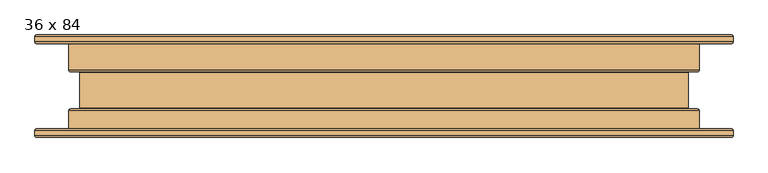
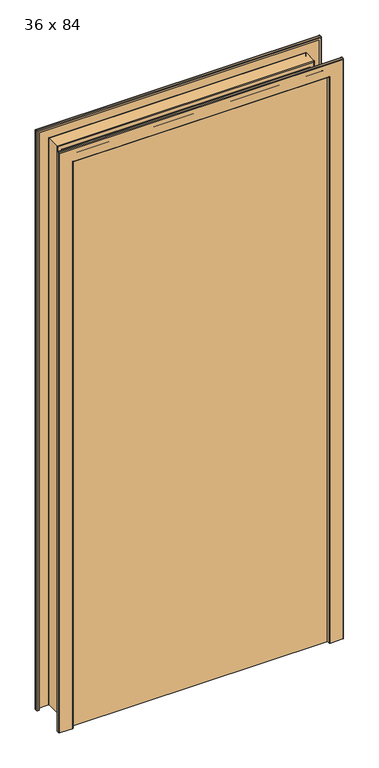
"""IFC4 building model written with IfcOpenShell, lengths in millimetres: door geometry, Door-Dunbarton_Doors-Hollow_Metal_Core : 36 x 84."""

from ifc_helpers import new_model, si_unit, frame, origin, origin_with_axes, place, context, project, spatial, polyline, circle_curve, ellipse_curve, outline, extrude, source, transform, mapped, element, save
from ifc_brep_helpers import plane_surface, cylinder_surface, revolved_surface, advanced_brep


def door_36_x_84_91fbd793(model_context):
    return source(origin(), model_context, "Body", "SolidModel", [
        advanced_brep(
        [(-505.42825, 61.976, 0.0), (-508.0, 64.54775, 0.0), (-508.0, 72.0725, 0.0), (-505.42825, 74.64425, 0.0), (-459.77175, 74.64425, 0.0), (-457.2, 72.0725, 0.0), (-457.2, 23.27275, 0.0), (-456.184, 22.25675, 0.0), (-443.89675, 22.25675, 0.0), (-441.325, 19.685, 0.0), (-441.325, -32.1056, 0.0), (-443.89675, -34.67735, 0.0), (-456.184, -34.67735, 0.0), (-457.2, -35.69335, 0.0), (-457.2, -72.009, 0.0), (-459.77175, -74.58075, 0.0), (-505.42825, -74.58075, 0.0), (-508.0, -72.009, 0.0), (-508.0, -64.48425, 0.0), (-505.42825, -61.9125, 0.0), (-500.0625, -61.9125, 0.0), (-500.0625, -63.46825, 0.0), (-505.42825, -63.46825, 0.0), (-506.44425, -64.48425, 0.0), (-506.44425, -72.009, 0.0), (-505.42825, -73.025, 0.0), (-459.77175, -73.025, 0.0), (-458.75575, -72.009, 0.0), (-458.75575, -35.69335, 0.0), (-456.184, -33.1216, 0.0), (-443.89675, -33.1216, 0.0), (-442.88075, -32.1056, 0.0), (-442.88075, 19.685, 0.0), (-443.89675, 20.701, 0.0), (-456.184, 20.701, 0.0), (-458.75575, 23.27275, 0.0), (-458.75575, 72.0725, 0.0), (-459.77175, 73.0885, 0.0), (-505.42825, 73.0885, 0.0), (-506.44425, 72.0725, 0.0), (-506.44425, 64.54775, 0.0), (-505.42825, 63.53175, 0.0), (-500.0625, 63.53175, 0.0), (-500.0625, 61.976, 0.0), (-505.42825, 61.976, 2181.82825), (-508.0, 64.54775, 2184.4), (-508.0, 72.0725, 2184.4), (-505.42825, 74.64425, 2181.82825), (505.42825, 74.64425, 2181.82825), (505.42825, 74.64425, 0.0), (459.77175, 74.64425, 0.0), (459.77175, 74.64425, 2136.17175), (-459.77175, 74.64425, 2136.17175), (-457.2, 72.0725, 2133.6), (-457.2, 23.27275, 2133.6), (-456.184, 22.25675, 2132.584), (456.184, 22.25675, 2132.584), (456.184, 22.25675, 0.0), (443.89675, 22.25675, 0.0), (443.89675, 22.25675, 2120.29675), (-443.89675, 22.25675, 2120.29675), (-441.325, 19.685, 2117.725), (-441.325, -32.1056, 2117.725), (-443.89675, -34.67735, 2120.29675), (443.89675, -34.67735, 2120.29675), (443.89675, -34.67735, 0.0), (456.184, -34.67735, 0.0), (456.184, -34.67735, 2132.584), (-456.184, -34.67735, 2132.584), (-457.2, -35.69335, 2133.6), (-457.2, -72.009, 2133.6), (-459.77175, -74.58075, 2136.17175), (459.77175, -74.58075, 2136.17175), (459.77175, -74.58075, 0.0), (505.42825, -74.58075, 0.0), (505.42825, -74.58075, 2181.82825), (-505.42825, -74.58075, 2181.82825), (-508.0, -72.009, 2184.4), (-508.0, -64.48425, 2184.4), (-505.42825, -61.9125, 2181.82825), (505.42825, -61.9125, 2181.82825), (505.42825, -61.9125, 0.0), (500.0625, -61.9125, 0.0), (500.0625, -61.9125, 2176.4625), (-500.0625, -61.9125, 2176.4625), (-500.0625, -63.46825, 2176.4625), (500.0625, -63.46825, 2176.4625), (500.0625, -63.46825, 0.0), (505.42825, -63.46825, 0.0), (505.42825, -63.46825, 2181.82825), (-505.42825, -63.46825, 2181.82825), (-506.44425, -64.48425, 2182.84425), (-506.44425, -72.009, 2182.84425), (-505.42825, -73.025, 2181.82825), (505.42825, -73.025, 2181.82825), (505.42825, -73.025, 0.0), (459.77175, -73.025, 0.0), (459.77175, -73.025, 2136.17175), (-459.77175, -73.025, 2136.17175), (-458.75575, -72.009, 2135.15575), (-458.75575, -35.69335, 2135.15575), (-456.184, -33.1216, 2132.584), (456.184, -33.1216, 2132.584), (456.184, -33.1216, 0.0), (443.89675, -33.1216, 0.0), (443.89675, -33.1216, 2120.29675), (-443.89675, -33.1216, 2120.29675), (-442.88075, -32.1056, 2119.28075), (-442.88075, 19.685, 2119.28075), (-443.89675, 20.701, 2120.29675), (443.89675, 20.701, 2120.29675), (443.89675, 20.701, 0.0), (456.184, 20.701, 0.0), (456.184, 20.701, 2132.584), (-456.184, 20.701, 2132.584), (-458.75575, 23.27275, 2135.15575), (-458.75575, 72.0725, 2135.15575), (-459.77175, 73.0885, 2136.17175), (459.77175, 73.0885, 2136.17175), (459.77175, 73.0885, 0.0), (505.42825, 73.0885, 0.0), (505.42825, 73.0885, 2181.82825), (-505.42825, 73.0885, 2181.82825), (-506.44425, 72.0725, 2182.84425), (-506.44425, 64.54775, 2182.84425), (-505.42825, 63.53175, 2181.82825), (505.42825, 63.53175, 2181.82825), (505.42825, 63.53175, 0.0), (500.0625, 63.53175, 0.0), (500.0625, 63.53175, 2176.4625), (-500.0625, 63.53175, 2176.4625), (-500.0625, 61.976, 2176.4625), (500.0625, 61.976, 2176.4625), (500.0625, 61.976, 0.0), (505.42825, 61.976, 0.0), (505.42825, 61.976, 2181.82825), (508.0, 64.54775, 2184.4), (508.0, 72.0725, 2184.4), (457.2, 72.0725, 2133.6), (457.2, 23.27275, 2133.6), (441.325, 19.685, 2117.725), (441.325, -32.1056, 2117.725), (457.2, -35.69335, 2133.6), (457.2, -72.009, 2133.6), (508.0, -72.009, 2184.4), (508.0, -64.48425, 2184.4), (506.44425, -64.48425, 2182.84425), (506.44425, -72.009, 2182.84425), (458.75575, -72.009, 2135.15575), (458.75575, -35.69335, 2135.15575), (442.88075, -32.1056, 2119.28075), (442.88075, 19.685, 2119.28075), (458.75575, 23.27275, 2135.15575), (458.75575, 72.0725, 2135.15575), (506.44425, 72.0725, 2182.84425), (506.44425, 64.54775, 2182.84425), (506.44425, 64.54775, 0.0), (506.44425, 72.0725, 0.0), (458.75575, 72.0725, 0.0), (458.75575, 23.27275, 0.0), (442.88075, 19.685, 0.0), (442.88075, -32.1056, 0.0), (458.75575, -35.69335, 0.0), (458.75575, -72.009, 0.0), (506.44425, -72.009, 0.0), (506.44425, -64.48425, 0.0), (508.0, -64.48425, 0.0), (508.0, -72.009, 0.0), (457.2, -72.009, 0.0), (457.2, -35.69335, 0.0), (441.325, -32.1056, 0.0), (441.325, 19.685, 0.0), (457.2, 23.27275, 0.0), (457.2, 72.0725, 0.0), (508.0, 72.0725, 0.0), (508.0, 64.54775, 0.0)],
        [
            (0, 1, circle_curve(frame((-505.42825, 64.54775, 0.0), z_axis=(0.0, 0.0, -1.0), x_axis=(0.0, -1.0, 0.0)), 2.57175)),
            (1, 2),
            (2, 3, circle_curve(frame((-505.42825, 72.0725, 0.0), z_axis=(0.0, 0.0, -1.0), x_axis=(0.0, -1.0, 0.0)), 2.57175)),
            (3, 4),
            (4, 5, circle_curve(frame((-459.77175, 72.0725, 0.0), z_axis=(0.0, 0.0, -1.0), x_axis=(0.0, -1.0, 0.0)), 2.57175)),
            (5, 6),
            (6, 7, circle_curve(frame((-456.184, 23.27275, 0.0), z_axis=(0.0, 0.0, 1.0), x_axis=(0.0, -1.0, 0.0)), 1.016)),
            (7, 8),
            (8, 9, circle_curve(frame((-443.89675, 19.685, 0.0), z_axis=(0.0, 0.0, -1.0), x_axis=(0.0, -1.0, 0.0)), 2.57175)),
            (9, 10),
            (10, 11, circle_curve(frame((-443.89675, -32.1056, 0.0), z_axis=(0.0, 0.0, -1.0), x_axis=(0.0, -1.0, 0.0)), 2.57175)),
            (11, 12),
            (12, 13, circle_curve(frame((-456.184, -35.69335, 0.0), z_axis=(0.0, 0.0, 1.0), x_axis=(0.0, -1.0, 0.0)), 1.016)),
            (13, 14),
            (14, 15, circle_curve(frame((-459.77175, -72.009, 0.0), z_axis=(0.0, 0.0, -1.0), x_axis=(0.0, -1.0, 0.0)), 2.57175)),
            (15, 16),
            (16, 17, circle_curve(frame((-505.42825, -72.009, 0.0), z_axis=(0.0, 0.0, -1.0), x_axis=(0.0, -1.0, 0.0)), 2.57175)),
            (17, 18),
            (18, 19, circle_curve(frame((-505.42825, -64.48425, 0.0), z_axis=(0.0, 0.0, -1.0), x_axis=(0.0, -1.0, 0.0)), 2.57175)),
            (19, 20),
            (20, 21),
            (21, 22),
            (22, 23, circle_curve(frame((-505.42825, -64.48425, 0.0), z_axis=(0.0, 0.0, 1.0), x_axis=(0.0, -1.0, 0.0)), 1.016)),
            (23, 24),
            (24, 25, circle_curve(frame((-505.42825, -72.009, 0.0), z_axis=(0.0, 0.0, 1.0), x_axis=(0.0, -1.0, 0.0)), 1.016)),
            (25, 26),
            (26, 27, circle_curve(frame((-459.77175, -72.009, 0.0), z_axis=(0.0, 0.0, 1.0), x_axis=(0.0, -1.0, 0.0)), 1.016)),
            (27, 28),
            (28, 29, circle_curve(frame((-456.184, -35.69335, 0.0), z_axis=(0.0, 0.0, -1.0), x_axis=(0.0, -1.0, 0.0)), 2.57175)),
            (29, 30),
            (30, 31, circle_curve(frame((-443.89675, -32.1056, 0.0), z_axis=(0.0, 0.0, 1.0), x_axis=(0.0, -1.0, 0.0)), 1.016)),
            (31, 32),
            (32, 33, circle_curve(frame((-443.89675, 19.685, 0.0), z_axis=(0.0, 0.0, 1.0), x_axis=(0.0, -1.0, 0.0)), 1.016)),
            (33, 34),
            (34, 35, circle_curve(frame((-456.184, 23.27275, 0.0), z_axis=(0.0, 0.0, -1.0), x_axis=(0.0, -1.0, 0.0)), 2.57175)),
            (35, 36),
            (36, 37, circle_curve(frame((-459.77175, 72.0725, 0.0), z_axis=(0.0, 0.0, 1.0), x_axis=(0.0, -1.0, 0.0)), 1.016)),
            (37, 38),
            (38, 39, circle_curve(frame((-505.42825, 72.0725, 0.0), z_axis=(0.0, 0.0, 1.0), x_axis=(0.0, -1.0, 0.0)), 1.016)),
            (39, 40),
            (40, 41, circle_curve(frame((-505.42825, 64.54775, 0.0), z_axis=(0.0, 0.0, 1.0), x_axis=(0.0, -1.0, 0.0)), 1.016)),
            (41, 42),
            (42, 43),
            (43, 0),
            (0, 44),
            (44, 45, ellipse_curve(frame((-505.42825, 64.54775, 2181.82825), z_axis=(-0.7071067811865475, 0.0, -0.7071067811865475), x_axis=(0.7071067811865474, 0.0, -0.7071067811865476)), 3.6370037, 2.57175)),
            (45, 1),
            (45, 46),
            (46, 2),
            (46, 47, ellipse_curve(frame((-505.42825, 72.0725, 2181.82825), z_axis=(-0.7071067811865475, 0.0, -0.7071067811865475), x_axis=(0.7071067811865474, 0.0, -0.7071067811865476)), 3.6370037, 2.57175)),
            (47, 3),
            (47, 48),
            (48, 49),
            (49, 50),
            (50, 51),
            (51, 52),
            (52, 4),
            (52, 53, ellipse_curve(frame((-459.77175, 72.0725, 2136.17175), z_axis=(-0.7071067811865475, 0.0, -0.7071067811865475), x_axis=(0.7071067811865474, 0.0, -0.7071067811865476)), 3.6370037, 2.57175)),
            (53, 5),
            (53, 54),
            (54, 6),
            (54, 55, ellipse_curve(frame((-456.184, 23.27275, 2132.584), z_axis=(0.7071067811865475, 0.0, 0.7071067811865475), x_axis=(-0.7071067811865474, 0.0, 0.7071067811865476)), 1.436841, 1.016)),
            (55, 7),
            (55, 56),
            (56, 57),
            (57, 58),
            (58, 59),
            (59, 60),
            (60, 8),
            (60, 61, ellipse_curve(frame((-443.89675, 19.685, 2120.29675), z_axis=(-0.7071067811865475, 0.0, -0.7071067811865475), x_axis=(0.7071067811865474, 0.0, -0.7071067811865476)), 3.6370037, 2.57175)),
            (61, 9),
            (61, 62),
            (62, 10),
            (62, 63, ellipse_curve(frame((-443.89675, -32.1056, 2120.29675), z_axis=(-0.7071067811865475, 0.0, -0.7071067811865475), x_axis=(0.7071067811865474, 0.0, -0.7071067811865476)), 3.6370037, 2.57175)),
            (63, 11),
            (63, 64),
            (64, 65),
            (65, 66),
            (66, 67),
            (67, 68),
            (68, 12),
            (68, 69, ellipse_curve(frame((-456.184, -35.69335, 2132.584), z_axis=(0.7071067811865475, 0.0, 0.7071067811865475), x_axis=(-0.7071067811865474, 0.0, 0.7071067811865476)), 1.436841, 1.016)),
            (69, 13),
            (69, 70),
            (70, 14),
            (70, 71, ellipse_curve(frame((-459.77175, -72.009, 2136.17175), z_axis=(-0.7071067811865475, 0.0, -0.7071067811865475), x_axis=(0.7071067811865474, 0.0, -0.7071067811865476)), 3.6370037, 2.57175)),
            (71, 15),
            (71, 72),
            (72, 73),
            (73, 74),
            (74, 75),
            (75, 76),
            (76, 16),
            (76, 77, ellipse_curve(frame((-505.42825, -72.009, 2181.82825), z_axis=(-0.7071067811865475, 0.0, -0.7071067811865475), x_axis=(0.7071067811865474, 0.0, -0.7071067811865476)), 3.6370037, 2.57175)),
            (77, 17),
            (77, 78),
            (78, 18),
            (78, 79, ellipse_curve(frame((-505.42825, -64.48425, 2181.82825), z_axis=(-0.7071067811865475, 0.0, -0.7071067811865475), x_axis=(0.7071067811865474, 0.0, -0.7071067811865476)), 3.6370037, 2.57175)),
            (79, 19),
            (79, 80),
            (80, 81),
            (81, 82),
            (82, 83),
            (83, 84),
            (84, 20),
            (84, 85),
            (85, 21),
            (85, 86),
            (86, 87),
            (87, 88),
            (88, 89),
            (89, 90),
            (90, 22),
            (90, 91, ellipse_curve(frame((-505.42825, -64.48425, 2181.82825), z_axis=(0.7071067811865475, 0.0, 0.7071067811865475), x_axis=(-0.7071067811865474, 0.0, 0.7071067811865476)), 1.436841, 1.016)),
            (91, 23),
            (91, 92),
            (92, 24),
            (92, 93, ellipse_curve(frame((-505.42825, -72.009, 2181.82825), z_axis=(0.7071067811865475, 0.0, 0.7071067811865475), x_axis=(-0.7071067811865474, 0.0, 0.7071067811865476)), 1.436841, 1.016)),
            (93, 25),
            (93, 94),
            (94, 95),
            (95, 96),
            (96, 97),
            (97, 98),
            (98, 26),
            (98, 99, ellipse_curve(frame((-459.77175, -72.009, 2136.17175), z_axis=(0.7071067811865475, 0.0, 0.7071067811865475), x_axis=(-0.7071067811865474, 0.0, 0.7071067811865476)), 1.436841, 1.016)),
            (99, 27),
            (99, 100),
            (100, 28),
            (100, 101, ellipse_curve(frame((-456.184, -35.69335, 2132.584), z_axis=(-0.7071067811865475, 0.0, -0.7071067811865475), x_axis=(0.7071067811865474, 0.0, -0.7071067811865476)), 3.6370037, 2.57175)),
            (101, 29),
            (101, 102),
            (102, 103),
            (103, 104),
            (104, 105),
            (105, 106),
            (106, 30),
            (106, 107, ellipse_curve(frame((-443.89675, -32.1056, 2120.29675), z_axis=(0.7071067811865475, 0.0, 0.7071067811865475), x_axis=(-0.7071067811865474, 0.0, 0.7071067811865476)), 1.436841, 1.016)),
            (107, 31),
            (107, 108),
            (108, 32),
            (108, 109, ellipse_curve(frame((-443.89675, 19.685, 2120.29675), z_axis=(0.7071067811865475, 0.0, 0.7071067811865475), x_axis=(-0.7071067811865474, 0.0, 0.7071067811865476)), 1.436841, 1.016)),
            (109, 33),
            (109, 110),
            (110, 111),
            (111, 112),
            (112, 113),
            (113, 114),
            (114, 34),
            (114, 115, ellipse_curve(frame((-456.184, 23.27275, 2132.584), z_axis=(-0.7071067811865475, 0.0, -0.7071067811865475), x_axis=(0.7071067811865474, 0.0, -0.7071067811865476)), 3.6370037, 2.57175)),
            (115, 35),
            (115, 116),
            (116, 36),
            (116, 117, ellipse_curve(frame((-459.77175, 72.0725, 2136.17175), z_axis=(0.7071067811865475, 0.0, 0.7071067811865475), x_axis=(-0.7071067811865474, 0.0, 0.7071067811865476)), 1.436841, 1.016)),
            (117, 37),
            (117, 118),
            (118, 119),
            (119, 120),
            (120, 121),
            (121, 122),
            (122, 38),
            (122, 123, ellipse_curve(frame((-505.42825, 72.0725, 2181.82825), z_axis=(0.7071067811865475, 0.0, 0.7071067811865475), x_axis=(-0.7071067811865474, 0.0, 0.7071067811865476)), 1.436841, 1.016)),
            (123, 39),
            (123, 124),
            (124, 40),
            (124, 125, ellipse_curve(frame((-505.42825, 64.54775, 2181.82825), z_axis=(0.7071067811865475, 0.0, 0.7071067811865475), x_axis=(-0.7071067811865474, 0.0, 0.7071067811865476)), 1.436841, 1.016)),
            (125, 41),
            (125, 126),
            (126, 127),
            (127, 128),
            (128, 129),
            (129, 130),
            (130, 42),
            (130, 131),
            (131, 43),
            (131, 132),
            (132, 133),
            (133, 134),
            (134, 135),
            (135, 44),
            (135, 136, ellipse_curve(frame((505.42825, 64.54775, 2181.82825), z_axis=(-0.7071067811865475, 0.0, 0.7071067811865475), x_axis=(-0.7071067811865476, 0.0, -0.7071067811865474)), 3.6370037, 2.57175)),
            (136, 45),
            (136, 137),
            (137, 46),
            (137, 48, ellipse_curve(frame((505.42825, 72.0725, 2181.82825), z_axis=(-0.7071067811865475, 0.0, 0.7071067811865475), x_axis=(-0.7071067811865476, 0.0, -0.7071067811865474)), 3.6370037, 2.57175)),
            (51, 138, ellipse_curve(frame((459.77175, 72.0725, 2136.17175), z_axis=(-0.7071067811865475, 0.0, 0.7071067811865475), x_axis=(-0.7071067811865476, 0.0, -0.7071067811865474)), 3.6370037, 2.57175)),
            (138, 53),
            (138, 139),
            (139, 54),
            (139, 56, ellipse_curve(frame((456.184, 23.27275, 2132.584), z_axis=(0.7071067811865475, 0.0, -0.7071067811865475), x_axis=(0.7071067811865476, 0.0, 0.7071067811865474)), 1.436841, 1.016)),
            (59, 140, ellipse_curve(frame((443.89675, 19.685, 2120.29675), z_axis=(-0.7071067811865475, 0.0, 0.7071067811865475), x_axis=(-0.7071067811865476, 0.0, -0.7071067811865474)), 3.6370037, 2.57175)),
            (140, 61),
            (140, 141),
            (141, 62),
            (141, 64, ellipse_curve(frame((443.89675, -32.1056, 2120.29675), z_axis=(-0.7071067811865475, 0.0, 0.7071067811865475), x_axis=(-0.7071067811865476, 0.0, -0.7071067811865474)), 3.6370037, 2.57175)),
            (67, 142, ellipse_curve(frame((456.184, -35.69335, 2132.584), z_axis=(0.7071067811865475, 0.0, -0.7071067811865475), x_axis=(0.7071067811865476, 0.0, 0.7071067811865474)), 1.436841, 1.016)),
            (142, 69),
            (142, 143),
            (143, 70),
            (143, 72, ellipse_curve(frame((459.77175, -72.009, 2136.17175), z_axis=(-0.7071067811865475, 0.0, 0.7071067811865475), x_axis=(-0.7071067811865476, 0.0, -0.7071067811865474)), 3.6370037, 2.57175)),
            (75, 144, ellipse_curve(frame((505.42825, -72.009, 2181.82825), z_axis=(-0.7071067811865475, 0.0, 0.7071067811865475), x_axis=(-0.7071067811865476, 0.0, -0.7071067811865474)), 3.6370037, 2.57175)),
            (144, 77),
            (144, 145),
            (145, 78),
            (145, 80, ellipse_curve(frame((505.42825, -64.48425, 2181.82825), z_axis=(-0.7071067811865475, 0.0, 0.7071067811865475), x_axis=(-0.7071067811865476, 0.0, -0.7071067811865474)), 3.6370037, 2.57175)),
            (83, 86),
            (89, 146, ellipse_curve(frame((505.42825, -64.48425, 2181.82825), z_axis=(0.7071067811865475, 0.0, -0.7071067811865475), x_axis=(0.7071067811865476, 0.0, 0.7071067811865474)), 1.436841, 1.016)),
            (146, 91),
            (146, 147),
            (147, 92),
            (147, 94, ellipse_curve(frame((505.42825, -72.009, 2181.82825), z_axis=(0.7071067811865475, 0.0, -0.7071067811865475), x_axis=(0.7071067811865476, 0.0, 0.7071067811865474)), 1.436841, 1.016)),
            (97, 148, ellipse_curve(frame((459.77175, -72.009, 2136.17175), z_axis=(0.7071067811865475, 0.0, -0.7071067811865475), x_axis=(0.7071067811865476, 0.0, 0.7071067811865474)), 1.436841, 1.016)),
            (148, 99),
            (148, 149),
            (149, 100),
            (149, 102, ellipse_curve(frame((456.184, -35.69335, 2132.584), z_axis=(-0.7071067811865475, 0.0, 0.7071067811865475), x_axis=(-0.7071067811865476, 0.0, -0.7071067811865474)), 3.6370037, 2.57175)),
            (105, 150, ellipse_curve(frame((443.89675, -32.1056, 2120.29675), z_axis=(0.7071067811865475, 0.0, -0.7071067811865475), x_axis=(0.7071067811865476, 0.0, 0.7071067811865474)), 1.436841, 1.016)),
            (150, 107),
            (150, 151),
            (151, 108),
            (151, 110, ellipse_curve(frame((443.89675, 19.685, 2120.29675), z_axis=(0.7071067811865475, 0.0, -0.7071067811865475), x_axis=(0.7071067811865476, 0.0, 0.7071067811865474)), 1.436841, 1.016)),
            (113, 152, ellipse_curve(frame((456.184, 23.27275, 2132.584), z_axis=(-0.7071067811865475, 0.0, 0.7071067811865475), x_axis=(-0.7071067811865476, 0.0, -0.7071067811865474)), 3.6370037, 2.57175)),
            (152, 115),
            (152, 153),
            (153, 116),
            (153, 118, ellipse_curve(frame((459.77175, 72.0725, 2136.17175), z_axis=(0.7071067811865475, 0.0, -0.7071067811865475), x_axis=(0.7071067811865476, 0.0, 0.7071067811865474)), 1.436841, 1.016)),
            (121, 154, ellipse_curve(frame((505.42825, 72.0725, 2181.82825), z_axis=(0.7071067811865475, 0.0, -0.7071067811865475), x_axis=(0.7071067811865476, 0.0, 0.7071067811865474)), 1.436841, 1.016)),
            (154, 123),
            (154, 155),
            (155, 124),
            (155, 126, ellipse_curve(frame((505.42825, 64.54775, 2181.82825), z_axis=(0.7071067811865475, 0.0, -0.7071067811865475), x_axis=(0.7071067811865476, 0.0, 0.7071067811865474)), 1.436841, 1.016)),
            (129, 132),
            (133, 128),
            (127, 156, circle_curve(frame((505.42825, 64.54775, 0.0), z_axis=(0.0, 0.0, 1.0), x_axis=(0.0, -1.0, 0.0)), 1.016)),
            (156, 157),
            (157, 120, circle_curve(frame((505.42825, 72.0725, 0.0), z_axis=(0.0, 0.0, 1.0), x_axis=(0.0, -1.0, 0.0)), 1.016)),
            (119, 158, circle_curve(frame((459.77175, 72.0725, 0.0), z_axis=(0.0, 0.0, 1.0), x_axis=(0.0, -1.0, 0.0)), 1.016)),
            (158, 159),
            (159, 112, circle_curve(frame((456.184, 23.27275, 0.0), z_axis=(0.0, 0.0, -1.0), x_axis=(0.0, -1.0, 0.0)), 2.57175)),
            (111, 160, circle_curve(frame((443.89675, 19.685, 0.0), z_axis=(0.0, 0.0, 1.0), x_axis=(0.0, -1.0, 0.0)), 1.016)),
            (160, 161),
            (161, 104, circle_curve(frame((443.89675, -32.1056, 0.0), z_axis=(0.0, 0.0, 1.0), x_axis=(0.0, -1.0, 0.0)), 1.016)),
            (103, 162, circle_curve(frame((456.184, -35.69335, 0.0), z_axis=(0.0, 0.0, -1.0), x_axis=(0.0, -1.0, 0.0)), 2.57175)),
            (162, 163),
            (163, 96, circle_curve(frame((459.77175, -72.009, 0.0), z_axis=(0.0, 0.0, 1.0), x_axis=(0.0, -1.0, 0.0)), 1.016)),
            (95, 164, circle_curve(frame((505.42825, -72.009, 0.0), z_axis=(0.0, 0.0, 1.0), x_axis=(0.0, -1.0, 0.0)), 1.016)),
            (164, 165),
            (165, 88, circle_curve(frame((505.42825, -64.48425, 0.0), z_axis=(0.0, 0.0, 1.0), x_axis=(0.0, -1.0, 0.0)), 1.016)),
            (87, 82),
            (81, 166, circle_curve(frame((505.42825, -64.48425, 0.0), z_axis=(0.0, 0.0, -1.0), x_axis=(0.0, -1.0, 0.0)), 2.57175)),
            (166, 167),
            (167, 74, circle_curve(frame((505.42825, -72.009, 0.0), z_axis=(0.0, 0.0, -1.0), x_axis=(0.0, -1.0, 0.0)), 2.57175)),
            (73, 168, circle_curve(frame((459.77175, -72.009, 0.0), z_axis=(0.0, 0.0, -1.0), x_axis=(0.0, -1.0, 0.0)), 2.57175)),
            (168, 169),
            (169, 66, circle_curve(frame((456.184, -35.69335, 0.0), z_axis=(0.0, 0.0, 1.0), x_axis=(0.0, -1.0, 0.0)), 1.016)),
            (65, 170, circle_curve(frame((443.89675, -32.1056, 0.0), z_axis=(0.0, 0.0, -1.0), x_axis=(0.0, -1.0, 0.0)), 2.57175)),
            (170, 171),
            (171, 58, circle_curve(frame((443.89675, 19.685, 0.0), z_axis=(0.0, 0.0, -1.0), x_axis=(0.0, -1.0, 0.0)), 2.57175)),
            (57, 172, circle_curve(frame((456.184, 23.27275, 0.0), z_axis=(0.0, 0.0, 1.0), x_axis=(0.0, -1.0, 0.0)), 1.016)),
            (172, 173),
            (173, 50, circle_curve(frame((459.77175, 72.0725, 0.0), z_axis=(0.0, 0.0, -1.0), x_axis=(0.0, -1.0, 0.0)), 2.57175)),
            (49, 174, circle_curve(frame((505.42825, 72.0725, 0.0), z_axis=(0.0, 0.0, -1.0), x_axis=(0.0, -1.0, 0.0)), 2.57175)),
            (174, 175),
            (175, 134, circle_curve(frame((505.42825, 64.54775, 0.0), z_axis=(0.0, 0.0, -1.0), x_axis=(0.0, -1.0, 0.0)), 2.57175)),
            (175, 136),
            (174, 137),
            (173, 138),
            (172, 139),
            (171, 140),
            (170, 141),
            (169, 142),
            (168, 143),
            (167, 144),
            (166, 145),
            (165, 146),
            (164, 147),
            (163, 148),
            (162, 149),
            (161, 150),
            (160, 151),
            (159, 152),
            (158, 153),
            (157, 154),
            (156, 155),
        ],
        [
            plane_surface(frame((-468.3125, -61.9125, 0.0), z_axis=(0.0, 0.0, -1.0), x_axis=(1.0, 0.0, 0.0))),
            cylinder_surface(frame((-505.42825, 64.54775, 0.0), z_axis=(0.0, 0.0, -1.0), x_axis=(0.0, -1.0, 0.0)), 2.57175),
            plane_surface(frame((-508.0, 64.54775, 0.0), z_axis=(-1.0, 0.0, 0.0), x_axis=(0.0, 0.0, 1.0))),
            cylinder_surface(frame((-505.42825, 72.0725, 0.0), z_axis=(0.0, 0.0, -1.0), x_axis=(0.0, -1.0, 0.0)), 2.57175),
            plane_surface(frame((-505.42825, 74.64425, 0.0), z_axis=(0.0, 1.0, 0.0), x_axis=(0.0, 0.0, 1.0))),
            cylinder_surface(frame((-459.77175, 72.0725, 0.0), z_axis=(0.0, 0.0, -1.0), x_axis=(0.0, -1.0, 0.0)), 2.57175),
            plane_surface(frame((-457.2, 72.0725, 0.0), z_axis=(1.0, 0.0, 0.0), x_axis=(0.0, 0.0, 1.0))),
            revolved_surface(polyline([(-456.184, 22.256749999999997, 2133.600000014587), (-456.184, 22.256749999999997, 0.0)]), (-456.184, 23.27275, 0.0), (0.0, 0.0, 1.0)),
            plane_surface(frame((-456.184, 22.25675, 0.0), z_axis=(0.0, 1.0, 0.0), x_axis=(0.0, 0.0, 1.0))),
            cylinder_surface(frame((-443.89675, 19.685, 0.0), z_axis=(0.0, 0.0, -1.0), x_axis=(0.0, -1.0, 0.0)), 2.57175),
            plane_surface(frame((-441.325, 19.685, 0.0), z_axis=(1.0, 0.0, 0.0), x_axis=(0.0, 0.0, 1.0))),
            cylinder_surface(frame((-443.89675, -32.1056, 0.0), z_axis=(0.0, 0.0, -1.0), x_axis=(0.0, -1.0, 0.0)), 2.57175),
            plane_surface(frame((-443.89675, -34.67735, 0.0), z_axis=(0.0, -1.0, 0.0), x_axis=(0.0, 0.0, 1.0))),
            revolved_surface(polyline([(-456.184, -36.70935, 2133.600000014587), (-456.184, -36.70935, 0.0)]), (-456.184, -35.69335, 0.0), (0.0, 0.0, 1.0)),
            plane_surface(frame((-457.2, -35.69335, 0.0), z_axis=(1.0, 0.0, 0.0), x_axis=(0.0, 0.0, 1.0))),
            cylinder_surface(frame((-459.77175, -72.009, 0.0), z_axis=(0.0, 0.0, -1.0), x_axis=(0.0, -1.0, 0.0)), 2.57175),
            plane_surface(frame((-459.77175, -74.58075, 0.0), z_axis=(0.0, -1.0, 0.0), x_axis=(0.0, 0.0, 1.0))),
            cylinder_surface(frame((-505.42825, -72.009, 0.0), z_axis=(0.0, 0.0, -1.0), x_axis=(0.0, -1.0, 0.0)), 2.57175),
            plane_surface(frame((-508.0, -72.009, 0.0), z_axis=(-1.0, 0.0, 0.0), x_axis=(0.0, 0.0, 1.0))),
            cylinder_surface(frame((-505.42825, -64.48425, 0.0), z_axis=(0.0, 0.0, -1.0), x_axis=(0.0, -1.0, 0.0)), 2.57175),
            plane_surface(frame((-505.42825, -61.9125, 0.0), z_axis=(0.0, 1.0, 0.0), x_axis=(0.0, 0.0, 1.0))),
            plane_surface(frame((-500.0625, -61.9125, 0.0), z_axis=(1.0, 0.0, 0.0), x_axis=(0.0, 0.0, 1.0))),
            plane_surface(frame((-500.0625, -63.46825, 0.0), z_axis=(0.0, -1.0, 0.0), x_axis=(0.0, 0.0, 1.0))),
            revolved_surface(polyline([(-505.42825, -65.50025000000001, 2182.844250014587), (-505.42825, -65.50025000000001, 0.0)]), (-505.42825, -64.48425, 0.0), (0.0, 0.0, 1.0)),
            plane_surface(frame((-506.44425, -64.48425, 0.0), z_axis=(1.0, 0.0, 0.0), x_axis=(0.0, 0.0, 1.0))),
            revolved_surface(polyline([(-505.42825, -73.025, 2182.844250014587), (-505.42825, -73.025, 0.0)]), (-505.42825, -72.009, 0.0), (0.0, 0.0, 1.0)),
            plane_surface(frame((-505.42825, -73.025, 0.0), z_axis=(0.0, 1.0, 0.0), x_axis=(0.0, 0.0, 1.0))),
            revolved_surface(polyline([(-459.77175, -73.025, 2137.187750014587), (-459.77175, -73.025, 0.0)]), (-459.77175, -72.009, 0.0), (0.0, 0.0, 1.0)),
            plane_surface(frame((-458.75575, -72.009, 0.0), z_axis=(-1.0, 0.0, 0.0), x_axis=(0.0, 0.0, 1.0))),
            cylinder_surface(frame((-456.184, -35.69335, 0.0), z_axis=(0.0, 0.0, -1.0), x_axis=(0.0, -1.0, 0.0)), 2.57175),
            plane_surface(frame((-456.184, -33.1216, 0.0), z_axis=(0.0, 1.0, 0.0), x_axis=(0.0, 0.0, 1.0))),
            revolved_surface(polyline([(-443.89675, -33.1216, 2121.312750014587), (-443.89675, -33.1216, 0.0)]), (-443.89675, -32.1056, 0.0), (0.0, 0.0, 1.0)),
            plane_surface(frame((-442.88075, -32.1056, 0.0), z_axis=(-1.0, 0.0, 0.0), x_axis=(0.0, 0.0, 1.0))),
            revolved_surface(polyline([(-443.89675, 18.668999999999997, 2121.312750014587), (-443.89675, 18.668999999999997, 0.0)]), (-443.89675, 19.685, 0.0), (0.0, 0.0, 1.0)),
            plane_surface(frame((-443.89675, 20.701, 0.0), z_axis=(0.0, -1.0, 0.0), x_axis=(0.0, 0.0, 1.0))),
            cylinder_surface(frame((-456.184, 23.27275, 0.0), z_axis=(0.0, 0.0, -1.0), x_axis=(0.0, -1.0, 0.0)), 2.57175),
            plane_surface(frame((-458.75575, 23.27275, 0.0), z_axis=(-1.0, 0.0, 0.0), x_axis=(0.0, 0.0, 1.0))),
            revolved_surface(polyline([(-459.77175, 71.0565, 2137.187750014587), (-459.77175, 71.0565, 0.0)]), (-459.77175, 72.0725, 0.0), (0.0, 0.0, 1.0)),
            plane_surface(frame((-459.77175, 73.0885, 0.0), z_axis=(0.0, -1.0, 0.0), x_axis=(0.0, 0.0, 1.0))),
            revolved_surface(polyline([(-505.42825, 71.0565, 2182.844250014587), (-505.42825, 71.0565, 0.0)]), (-505.42825, 72.0725, 0.0), (0.0, 0.0, 1.0)),
            plane_surface(frame((-506.44425, 72.0725, 0.0), z_axis=(1.0, 0.0, 0.0), x_axis=(0.0, 0.0, 1.0))),
            revolved_surface(polyline([(-505.42825, 63.531749999999995, 2182.844250014587), (-505.42825, 63.531749999999995, 0.0)]), (-505.42825, 64.54775, 0.0), (0.0, 0.0, 1.0)),
            plane_surface(frame((-505.42825, 63.53175, 0.0), z_axis=(0.0, 1.0, 0.0), x_axis=(0.0, 0.0, 1.0))),
            plane_surface(frame((-500.0625, 63.53175, 0.0), z_axis=(1.0, 0.0, 0.0), x_axis=(0.0, 0.0, 1.0))),
            plane_surface(frame((-500.0625, 61.976, 0.0), z_axis=(0.0, -1.0, 0.0), x_axis=(0.0, 0.0, 1.0))),
            cylinder_surface(frame((-468.3125, 64.54775, 2181.82825), z_axis=(-1.0, 0.0, 0.0), x_axis=(0.0, -1.0, 0.0)), 2.57175),
            plane_surface(frame((-508.0, 64.54775, 2184.4), z_axis=(0.0, 0.0, 1.0), x_axis=(1.0, 0.0, 0.0))),
            cylinder_surface(frame((-468.3125, 72.0725, 2181.82825), z_axis=(-1.0, 0.0, 0.0), x_axis=(0.0, -1.0, 0.0)), 2.57175),
            cylinder_surface(frame((-468.3125, 72.0725, 2136.17175), z_axis=(-1.0, 0.0, 0.0), x_axis=(0.0, -1.0, 0.0)), 2.57175),
            plane_surface(frame((-457.2, 72.0725, 2133.6), z_axis=(0.0, 0.0, -1.0), x_axis=(1.0, 0.0, 0.0))),
            revolved_surface(polyline([(457.20000001458686, 22.256749999999997, 2132.584), (-457.20000001458686, 22.256749999999997, 2132.584)]), (-468.3125, 23.27275, 2132.584), (1.0, 0.0, 0.0)),
            cylinder_surface(frame((-468.3125, 19.685, 2120.29675), z_axis=(-1.0, 0.0, 0.0), x_axis=(0.0, -1.0, 0.0)), 2.57175),
            plane_surface(frame((-441.325, 19.685, 2117.725), z_axis=(0.0, 0.0, -1.0), x_axis=(1.0, 0.0, 0.0))),
            cylinder_surface(frame((-468.3125, -32.1056, 2120.29675), z_axis=(-1.0, 0.0, 0.0), x_axis=(0.0, -1.0, 0.0)), 2.57175),
            revolved_surface(polyline([(457.20000001458686, -36.70935, 2132.584), (-457.20000001458686, -36.70935, 2132.584)]), (-468.3125, -35.69335, 2132.584), (1.0, 0.0, 0.0)),
            plane_surface(frame((-457.2, -35.69335, 2133.6), z_axis=(0.0, 0.0, -1.0), x_axis=(1.0, 0.0, 0.0))),
            cylinder_surface(frame((-468.3125, -72.009, 2136.17175), z_axis=(-1.0, 0.0, 0.0), x_axis=(0.0, -1.0, 0.0)), 2.57175),
            cylinder_surface(frame((-468.3125, -72.009, 2181.82825), z_axis=(-1.0, 0.0, 0.0), x_axis=(0.0, -1.0, 0.0)), 2.57175),
            plane_surface(frame((-508.0, -72.009, 2184.4), z_axis=(0.0, 0.0, 1.0), x_axis=(1.0, 0.0, 0.0))),
            cylinder_surface(frame((-468.3125, -64.48425, 2181.82825), z_axis=(-1.0, 0.0, 0.0), x_axis=(0.0, -1.0, 0.0)), 2.57175),
            plane_surface(frame((-500.0625, -61.9125, 2176.4625), z_axis=(0.0, 0.0, -1.0), x_axis=(1.0, 0.0, 0.0))),
            revolved_surface(polyline([(506.4442500145868, -65.50025000000001, 2181.82825), (-506.4442500145868, -65.50025000000001, 2181.82825)]), (-468.3125, -64.48425, 2181.82825), (1.0, 0.0, 0.0)),
            plane_surface(frame((-506.44425, -64.48425, 2182.84425), z_axis=(0.0, 0.0, -1.0), x_axis=(1.0, 0.0, 0.0))),
            revolved_surface(polyline([(506.4442500145868, -73.025, 2181.82825), (-506.4442500145868, -73.025, 2181.82825)]), (-468.3125, -72.009, 2181.82825), (1.0, 0.0, 0.0)),
            revolved_surface(polyline([(460.7877500145869, -73.025, 2136.17175), (-460.78775001458683, -73.025, 2136.17175)]), (-468.3125, -72.009, 2136.17175), (1.0, 0.0, 0.0)),
            plane_surface(frame((-458.75575, -72.009, 2135.15575), z_axis=(0.0, 0.0, 1.0), x_axis=(1.0, 0.0, 0.0))),
            cylinder_surface(frame((-468.3125, -35.69335, 2132.584), z_axis=(-1.0, 0.0, 0.0), x_axis=(0.0, -1.0, 0.0)), 2.57175),
            revolved_surface(polyline([(444.9127500145869, -33.1216, 2120.29675), (-444.91275001458683, -33.1216, 2120.29675)]), (-468.3125, -32.1056, 2120.29675), (1.0, 0.0, 0.0)),
            plane_surface(frame((-442.88075, -32.1056, 2119.28075), z_axis=(0.0, 0.0, 1.0), x_axis=(1.0, 0.0, 0.0))),
            revolved_surface(polyline([(444.9127500145869, 18.668999999999997, 2120.29675), (-444.91275001458683, 18.668999999999997, 2120.29675)]), (-468.3125, 19.685, 2120.29675), (1.0, 0.0, 0.0)),
            cylinder_surface(frame((-468.3125, 23.27275, 2132.584), z_axis=(-1.0, 0.0, 0.0), x_axis=(0.0, -1.0, 0.0)), 2.57175),
            plane_surface(frame((-458.75575, 23.27275, 2135.15575), z_axis=(0.0, 0.0, 1.0), x_axis=(1.0, 0.0, 0.0))),
            revolved_surface(polyline([(460.7877500145869, 71.0565, 2136.17175), (-460.78775001458683, 71.0565, 2136.17175)]), (-468.3125, 72.0725, 2136.17175), (1.0, 0.0, 0.0)),
            revolved_surface(polyline([(506.4442500145868, 71.0565, 2181.82825), (-506.4442500145868, 71.0565, 2181.82825)]), (-468.3125, 72.0725, 2181.82825), (1.0, 0.0, 0.0)),
            plane_surface(frame((-506.44425, 72.0725, 2182.84425), z_axis=(0.0, 0.0, -1.0), x_axis=(1.0, 0.0, 0.0))),
            revolved_surface(polyline([(506.4442500145868, 63.531749999999995, 2181.82825), (-506.4442500145868, 63.531749999999995, 2181.82825)]), (-468.3125, 64.54775, 2181.82825), (1.0, 0.0, 0.0)),
            plane_surface(frame((-500.0625, 63.53175, 2176.4625), z_axis=(0.0, 0.0, -1.0), x_axis=(1.0, 0.0, 0.0))),
            plane_surface(frame((468.3125, -61.9125, 0.0), z_axis=(0.0, 0.0, -1.0), x_axis=(-1.0, 0.0, 0.0))),
            cylinder_surface(frame((505.42825, 64.54775, 2144.7125), z_axis=(0.0, 0.0, 1.0), x_axis=(0.0, -1.0, 0.0)), 2.57175),
            plane_surface(frame((508.0, 64.54775, 2184.4), z_axis=(1.0, 0.0, 0.0), x_axis=(0.0, 0.0, -1.0))),
            cylinder_surface(frame((505.42825, 72.0725, 2144.7125), z_axis=(0.0, 0.0, 1.0), x_axis=(0.0, -1.0, 0.0)), 2.57175),
            cylinder_surface(frame((459.77175, 72.0725, 2144.7125), z_axis=(0.0, 0.0, 1.0), x_axis=(0.0, -1.0, 0.0)), 2.57175),
            plane_surface(frame((457.2, 72.0725, 2133.6), z_axis=(-1.0, 0.0, 0.0), x_axis=(0.0, 0.0, -1.0))),
            revolved_surface(polyline([(456.184, 22.256749999999997, 0.0), (456.184, 22.256749999999997, 2133.600000014587)]), (456.184, 23.27275, 2144.7125), (0.0, 0.0, -1.0)),
            cylinder_surface(frame((443.89675, 19.685, 2144.7125), z_axis=(0.0, 0.0, 1.0), x_axis=(0.0, -1.0, 0.0)), 2.57175),
            plane_surface(frame((441.325, 19.685, 2117.725), z_axis=(-1.0, 0.0, 0.0), x_axis=(0.0, 0.0, -1.0))),
            cylinder_surface(frame((443.89675, -32.1056, 2144.7125), z_axis=(0.0, 0.0, 1.0), x_axis=(0.0, -1.0, 0.0)), 2.57175),
            revolved_surface(polyline([(456.184, -36.70935, 0.0), (456.184, -36.70935, 2133.600000014587)]), (456.184, -35.69335, 2144.7125), (0.0, 0.0, -1.0)),
            plane_surface(frame((457.2, -35.69335, 2133.6), z_axis=(-1.0, 0.0, 0.0), x_axis=(0.0, 0.0, -1.0))),
            cylinder_surface(frame((459.77175, -72.009, 2144.7125), z_axis=(0.0, 0.0, 1.0), x_axis=(0.0, -1.0, 0.0)), 2.57175),
            cylinder_surface(frame((505.42825, -72.009, 2144.7125), z_axis=(0.0, 0.0, 1.0), x_axis=(0.0, -1.0, 0.0)), 2.57175),
            plane_surface(frame((508.0, -72.009, 2184.4), z_axis=(1.0, 0.0, 0.0), x_axis=(0.0, 0.0, -1.0))),
            cylinder_surface(frame((505.42825, -64.48425, 2144.7125), z_axis=(0.0, 0.0, 1.0), x_axis=(0.0, -1.0, 0.0)), 2.57175),
            plane_surface(frame((500.0625, -61.9125, 2176.4625), z_axis=(-1.0, 0.0, 0.0), x_axis=(0.0, 0.0, -1.0))),
            revolved_surface(polyline([(505.42825, -65.50025000000001, 0.0), (505.42825, -65.50025000000001, 2182.844250014587)]), (505.42825, -64.48425, 2144.7125), (0.0, 0.0, -1.0)),
            plane_surface(frame((506.44425, -64.48425, 2182.84425), z_axis=(-1.0, 0.0, 0.0), x_axis=(0.0, 0.0, -1.0))),
            revolved_surface(polyline([(505.42825, -73.025, 0.0), (505.42825, -73.025, 2182.844250014587)]), (505.42825, -72.009, 2144.7125), (0.0, 0.0, -1.0)),
            revolved_surface(polyline([(459.77175, -73.025, 0.0), (459.77175, -73.025, 2137.187750014587)]), (459.77175, -72.009, 2144.7125), (0.0, 0.0, -1.0)),
            plane_surface(frame((458.75575, -72.009, 2135.15575), z_axis=(1.0, 0.0, 0.0), x_axis=(0.0, 0.0, -1.0))),
            cylinder_surface(frame((456.184, -35.69335, 2144.7125), z_axis=(0.0, 0.0, 1.0), x_axis=(0.0, -1.0, 0.0)), 2.57175),
            revolved_surface(polyline([(443.89675, -33.1216, 0.0), (443.89675, -33.1216, 2121.312750014587)]), (443.89675, -32.1056, 2144.7125), (0.0, 0.0, -1.0)),
            plane_surface(frame((442.88075, -32.1056, 2119.28075), z_axis=(1.0, 0.0, 0.0), x_axis=(0.0, 0.0, -1.0))),
            revolved_surface(polyline([(443.89675, 18.668999999999997, 0.0), (443.89675, 18.668999999999997, 2121.312750014587)]), (443.89675, 19.685, 2144.7125), (0.0, 0.0, -1.0)),
            cylinder_surface(frame((456.184, 23.27275, 2144.7125), z_axis=(0.0, 0.0, 1.0), x_axis=(0.0, -1.0, 0.0)), 2.57175),
            plane_surface(frame((458.75575, 23.27275, 2135.15575), z_axis=(1.0, 0.0, 0.0), x_axis=(0.0, 0.0, -1.0))),
            revolved_surface(polyline([(459.77175, 71.0565, 0.0), (459.77175, 71.0565, 2137.187750014587)]), (459.77175, 72.0725, 2144.7125), (0.0, 0.0, -1.0)),
            revolved_surface(polyline([(505.42825, 71.0565, 0.0), (505.42825, 71.0565, 2182.844250014587)]), (505.42825, 72.0725, 2144.7125), (0.0, 0.0, -1.0)),
            plane_surface(frame((506.44425, 72.0725, 2182.84425), z_axis=(-1.0, 0.0, 0.0), x_axis=(0.0, 0.0, -1.0))),
            revolved_surface(polyline([(505.42825, 63.531749999999995, 0.0), (505.42825, 63.531749999999995, 2182.844250014587)]), (505.42825, 64.54775, 2144.7125), (0.0, 0.0, -1.0)),
            plane_surface(frame((500.0625, 63.53175, 2176.4625), z_axis=(-1.0, 0.0, 0.0), x_axis=(0.0, 0.0, -1.0))),
        ],
        [
            (0, [[1, 2, 3, 4, 5, 6, 7, 8, 9, 10, 11, 12, 13, 14, 15, 16, 17, 18, 19, 20, 21, 22, 23, 24, 25, 26, 27, 28, 29, 30, 31, 32, 33, 34, 35, 36, 37, 38, 39, 40, 41, 42, 43, 44]]),
            (1, [[-1, 45, 46, 47]]),
            (2, [[-2, -47, 48, 49]]),
            (3, [[-3, -49, 50, 51]]),
            (4, [[-4, -51, 52, 53, 54, 55, 56, 57]]),
            (5, [[-5, -57, 58, 59]]),
            (6, [[-6, -59, 60, 61]]),
            (7, [[-7, -61, 62, 63]]),
            (8, [[-8, -63, 64, 65, 66, 67, 68, 69]]),
            (9, [[-9, -69, 70, 71]]),
            (10, [[-10, -71, 72, 73]]),
            (11, [[-11, -73, 74, 75]]),
            (12, [[-12, -75, 76, 77, 78, 79, 80, 81]]),
            (13, [[-13, -81, 82, 83]]),
            (14, [[-14, -83, 84, 85]]),
            (15, [[-15, -85, 86, 87]]),
            (16, [[-16, -87, 88, 89, 90, 91, 92, 93]]),
            (17, [[-17, -93, 94, 95]]),
            (18, [[-18, -95, 96, 97]]),
            (19, [[-19, -97, 98, 99]]),
            (20, [[-20, -99, 100, 101, 102, 103, 104, 105]]),
            (21, [[-21, -105, 106, 107]]),
            (22, [[-22, -107, 108, 109, 110, 111, 112, 113]]),
            (23, [[-23, -113, 114, 115]]),
            (24, [[-24, -115, 116, 117]]),
            (25, [[-25, -117, 118, 119]]),
            (26, [[-26, -119, 120, 121, 122, 123, 124, 125]]),
            (27, [[-27, -125, 126, 127]]),
            (28, [[-28, -127, 128, 129]]),
            (29, [[-29, -129, 130, 131]]),
            (30, [[-30, -131, 132, 133, 134, 135, 136, 137]]),
            (31, [[-31, -137, 138, 139]]),
            (32, [[-32, -139, 140, 141]]),
            (33, [[-33, -141, 142, 143]]),
            (34, [[-34, -143, 144, 145, 146, 147, 148, 149]]),
            (35, [[-35, -149, 150, 151]]),
            (36, [[-36, -151, 152, 153]]),
            (37, [[-37, -153, 154, 155]]),
            (38, [[-38, -155, 156, 157, 158, 159, 160, 161]]),
            (39, [[-39, -161, 162, 163]]),
            (40, [[-40, -163, 164, 165]]),
            (41, [[-41, -165, 166, 167]]),
            (42, [[-42, -167, 168, 169, 170, 171, 172, 173]]),
            (43, [[-43, -173, 174, 175]]),
            (44, [[-44, -175, 176, 177, 178, 179, 180, -45]]),
            (45, [[-46, -180, 181, 182]]),
            (46, [[-48, -182, 183, 184]]),
            (47, [[-50, -184, 185, -52]]),
            (48, [[-58, -56, 186, 187]]),
            (49, [[-60, -187, 188, 189]]),
            (50, [[-62, -189, 190, -64]]),
            (51, [[-70, -68, 191, 192]]),
            (52, [[-72, -192, 193, 194]]),
            (53, [[-74, -194, 195, -76]]),
            (54, [[-82, -80, 196, 197]]),
            (55, [[-84, -197, 198, 199]]),
            (56, [[-86, -199, 200, -88]]),
            (57, [[-94, -92, 201, 202]]),
            (58, [[-96, -202, 203, 204]]),
            (59, [[-98, -204, 205, -100]]),
            (60, [[-106, -104, 206, -108]]),
            (61, [[-114, -112, 207, 208]]),
            (62, [[-116, -208, 209, 210]]),
            (63, [[-118, -210, 211, -120]]),
            (64, [[-126, -124, 212, 213]]),
            (65, [[-128, -213, 214, 215]]),
            (66, [[-130, -215, 216, -132]]),
            (67, [[-138, -136, 217, 218]]),
            (68, [[-140, -218, 219, 220]]),
            (69, [[-142, -220, 221, -144]]),
            (70, [[-150, -148, 222, 223]]),
            (71, [[-152, -223, 224, 225]]),
            (72, [[-154, -225, 226, -156]]),
            (73, [[-162, -160, 227, 228]]),
            (74, [[-164, -228, 229, 230]]),
            (75, [[-166, -230, 231, -168]]),
            (76, [[-174, -172, 232, -176]]),
            (77, [[-178, 233, -170, 234, 235, 236, -158, 237, 238, 239, -146, 240, 241, 242, -134, 243, 244, 245, -122, 246, 247, 248, -110, 249, -102, 250, 251, 252, -90, 253, 254, 255, -78, 256, 257, 258, -66, 259, 260, 261, -54, 262, 263, 264]]),
            (78, [[-181, -179, -264, 265]]),
            (79, [[-183, -265, -263, 266]]),
            (80, [[-185, -266, -262, -53]]),
            (81, [[-186, -55, -261, 267]]),
            (82, [[-188, -267, -260, 268]]),
            (83, [[-190, -268, -259, -65]]),
            (84, [[-191, -67, -258, 269]]),
            (85, [[-193, -269, -257, 270]]),
            (86, [[-195, -270, -256, -77]]),
            (87, [[-196, -79, -255, 271]]),
            (88, [[-198, -271, -254, 272]]),
            (89, [[-200, -272, -253, -89]]),
            (90, [[-201, -91, -252, 273]]),
            (91, [[-203, -273, -251, 274]]),
            (92, [[-205, -274, -250, -101]]),
            (93, [[-206, -103, -249, -109]]),
            (94, [[-207, -111, -248, 275]]),
            (95, [[-209, -275, -247, 276]]),
            (96, [[-211, -276, -246, -121]]),
            (97, [[-212, -123, -245, 277]]),
            (98, [[-214, -277, -244, 278]]),
            (99, [[-216, -278, -243, -133]]),
            (100, [[-217, -135, -242, 279]]),
            (101, [[-219, -279, -241, 280]]),
            (102, [[-221, -280, -240, -145]]),
            (103, [[-222, -147, -239, 281]]),
            (104, [[-224, -281, -238, 282]]),
            (105, [[-226, -282, -237, -157]]),
            (106, [[-227, -159, -236, 283]]),
            (107, [[-229, -283, -235, 284]]),
            (108, [[-231, -284, -234, -169]]),
            (109, [[-232, -171, -233, -177]]),
        ],
    ),
        extrude(outline(polyline([(455.64425, -35.69335), (455.64425, -61.9125), (-455.64425, -61.9125), (-455.64425, -35.69335), (455.64425, -35.69335)])), origin_with_axes(), (0.0, 0.0, 1.0), 2133.6),
    ])


if __name__ == "__main__":
    model = new_model("IFC4")
    model_context = context("Model", 3, world=origin())
    ifc_project = project(units=[si_unit("LENGTHUNIT", "METRE", prefix="MILLI")], contexts=[model_context])
    site = spatial("IfcSite", under=ifc_project)
    building = spatial("IfcBuilding", under=site)
    placement = place(None, origin())
    door_36_x_84_shape = door_36_x_84_91fbd793(model_context)
    element("IfcDoor", 1, ObjectType="Door-Dunbarton_Doors-Hollow_Metal_Core : 36 x 84", at=placement, inside=building, context=model_context, shape_type="MappedRepresentation", body=[
        mapped(door_36_x_84_shape, transform((0.0, 0.0, 0.0), x_axis=(1.0, 0.0, 0.0), y_axis=(0.0, 1.0, 0.0), z_axis=(0.0, 0.0, 1.0))),
    ])
    save(model, "model.ifc")

# Revit data of these elements
# Type "Door-Dunbarton_Doors-Hollow_Metal_Core : 36 x 84"
#   Type Mark = "15"
#   URL = "http://dunbarton.com/"
#   Product Page URL = "http://dunbarton.com/products/rediframe-door-frames/rediframe-hollow-metal/"
#   Product Name = "Hollow Metal Non Kerfed"
#   Product Documentation Link = "http://dunbarton.com/products/rediframe-door-frames/rediframe-drawings-overview/"
#   Model = "Non-Kerfed"
#   Material = ""
#   Manufacturer = "Dunbarton Corporation"
#   Description = "Hollow Metal Non-Kerfed Profile"
#   Frame Projection Ext. = 0' - 1"
#   Frame Projection Int. = 0' - 1"
#   Frame Width = 0' - 3"
#   Height = 7' - 0"
#   Width = 3' - 0"
#   Non-Kerfed = yes
#   Kerfed = no
#   Hollow Metal Casing = Metal-Dunbarton_Doors-White
#   Flush Door = Metal-Dunbarton_Doors-Aluminum
#   Function = (empty or 0)
#   Wall Closure = (empty or 0)
# Element 1 (IfcDoor, "Door-Dunbarton_Doors-Hollow_Metal_Core : 36 x 84")
#   Materials on its faces: "Metal-Dunbarton_Doors-White", "Metal-Dunbarton_Doors-Aluminum"
# Materials
#   "Metal-Dunbarton_Doors-White": class "Miscellaneous", colour RGB 230 233 236, transparency 0
#   "Metal-Dunbarton_Doors-Aluminum": class "System", colour RGB 143 142 141, transparency 0
